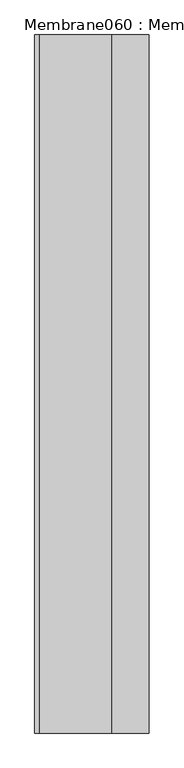
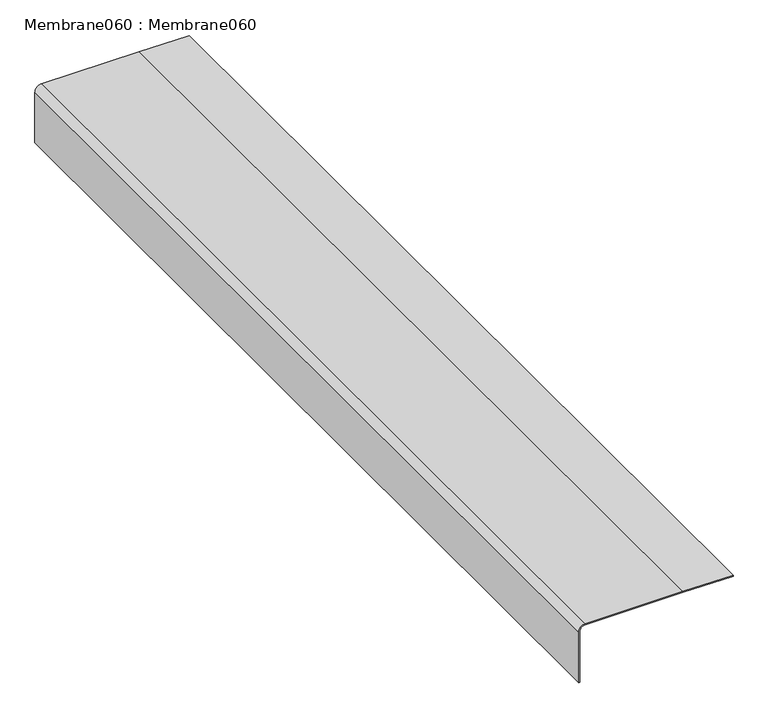
"""IFC4 building model written with IfcOpenShell, lengths in millimetres: proxy geometry, Membrane060 : Membrane060."""

from ifc_helpers import new_model, si_unit, point, frame, frame_2d, origin, place, context, project, spatial, polyline, circle_curve, trimmed, segment, composite_curve, outline, extrude, source, transform, mapped, element, save


def membrane060_membrane060_3178415f(model_context):
    return source(origin(), model_context, "Body", "SweptSolid", [
        extrude(outline(composite_curve([segment(trimmed(circle_curve(frame_2d((40234.5370749, -5013.558233)), 12.0), [point((40234.5370749, -5025.558233))], [point((40246.5370749, -5013.558233))], True, "CARTESIAN"), True, "CONTINUOUS"), segment(polyline([(40246.5370749, -5013.558233), (40246.5370749, -4806.2897295), (40245.0046252, -4699.8063764), (40247.0048323, -4699.8063764), (40248.5370749, -4806.2753388), (40248.5370749, -5013.558233)]), True, "CONTINUOUS"), segment(trimmed(circle_curve(frame_2d((40234.5370749, -5013.558233)), 14.0), [point((40248.5370749, -5013.558233))], [point((40234.5370749, -5027.558233))], False, "CARTESIAN"), True, "CONTINUOUS"), segment(polyline([(40234.5370749, -5027.558233), (40120.9129128, -5027.558233), (40120.9129128, -5025.558233), (40234.5370749, -5025.558233)]), True, "CONTINUOUS")], self_intersect=False)), frame((0.0, -1052.8906574, 0.0), z_axis=(0.0, 1.0, 0.0), x_axis=(0.0, 0.0, 1.0)), (0.0, 0.0, 1.0), 2000.0),
    ])


if __name__ == "__main__":
    model = new_model("IFC4")
    model_context = context("Model", 3, world=origin())
    ifc_project = project(units=[si_unit("LENGTHUNIT", "METRE", prefix="MILLI")], contexts=[model_context])
    site = spatial("IfcSite", under=ifc_project)
    building = spatial("IfcBuilding", under=site)
    placement = place(None, origin())
    membrane060_membrane060_shape = membrane060_membrane060_3178415f(model_context)
    element("IfcBuildingElementProxy", 1, Name="Membrane060 : Membrane060", ObjectType="Membrane060 : Membrane060", at=placement, inside=building, context=model_context, shape_type="MappedRepresentation", body=[
        mapped(membrane060_membrane060_shape, transform((0.0, 0.0, 0.0), x_axis=(1.0, 0.0, 0.0), y_axis=(0.0, 1.0, 0.0), z_axis=(0.0, 0.0, 1.0))),
    ])
    save(model, "model.ifc")

# Revit data of these elements
# Type "Membrane060 : Membrane060"
#   NameOverride = "Membrane060"
# Element 1 (IfcBuildingElementProxy, "Membrane060 : Membrane060")
#   Materials on its faces: "THREE PLY BUILT UP ROOF MEMBRANE"
# Materials
#   "THREE PLY BUILT UP ROOF MEMBRANE": class "Unassigned", colour RGB 63 63 63, transparency 0
